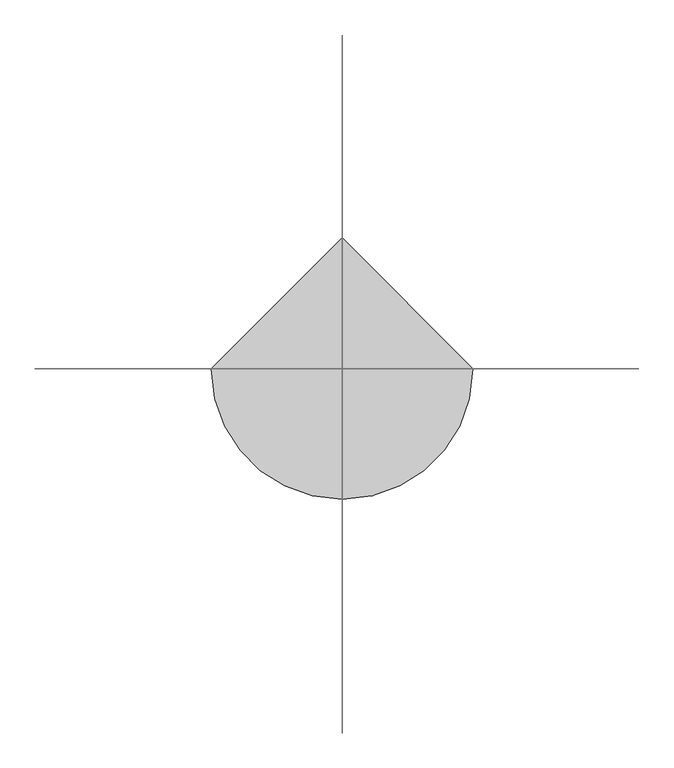
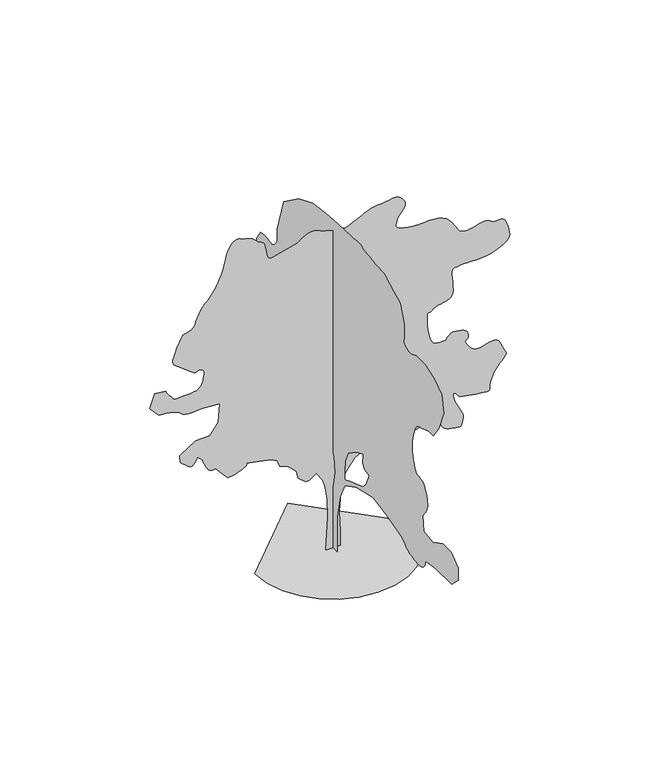
"""IFC4 building model written with IfcOpenShell, lengths in millimetres: geographic element geometry, RPC 木 - 落葉樹 : サンザシ - 7.4 メートル."""

from ifc_helpers import new_model, si_unit, origin, place, context, project, spatial, triangles, source, transform, mapped, element, save


def geographic_element_c28d403f(model_context):
    return source(origin(), model_context, "Body", "Tessellation", [
        triangles([(154.5387321, 0.0003833, 0.0187505), (-149.642156, 0.0003833, 0.0187505), (-106.1871776, 0.0003405, 717.0148825), (-117.051113, 0.0003185, 1086.3780928), (-160.5051012, 0.0003017, 1368.8308376), (-203.9600796, 0.0002913, 1542.6492977), (-345.1849986, 0.0002797, 1738.1941933), (-486.4138418, 0.0002855, 1640.4205101), (-562.4586551, 0.0002862, 1629.557365), (-714.5482452, 0.0002784, 1759.9204834), (-758.0034416, 0.000268, 1933.7389435), (-910.0929955, 0.000259, 2085.8284973), (-1094.7746733, 0.0002544, 2161.8732742), (-1149.0930147, 0.0002467, 2292.2365379), (-1268.5930607, 0.0002428, 2357.4181698), (-1518.4538269, 0.0002395, 2411.7365112), (-1768.3170639, 0.0002369, 2455.1893822), (-1766.353521, 0.0002375, 2445.7838516), (-1766.5756004, 0.0002381, 2435.806263), (-1771.1684887, 0.0002388, 2424.6889183), (-1782.3178082, 0.0002395, 2411.8623756), (-1802.2065651, 0.0002404, 2396.7539955), (-1833.0250328, 0.0002415, 2378.7966614), (-1876.9538921, 0.0002428, 2357.4181698), (-1925.9491573, 0.000244, 2336.6735058), (-1970.9560032, 0.000245, 2320.4872845), (-2012.6351452, 0.0002457, 2308.1046101), (-2051.6577633, 0.0002463, 2298.760849), (-2088.6823929, 0.0002467, 2291.6987801), (-2124.375127, 0.000247, 2286.1562405), (-2159.4067097, 0.0002473, 2281.3732475), (-2278.906683, 0.0002395, 2411.7365112), (-2409.2698013, 0.0002305, 2563.8260651), (-2434.8615532, 0.0002307, 2559.4600525), (-2460.3567993, 0.0002309, 2556.7959709), (-2485.6575806, 0.0002308, 2557.5607498), (-2510.6941338, 0.0002305, 2563.4560295), (-2535.3362343, 0.0002297, 2576.1840317), (-2559.4847603, 0.0002285, 2597.4713951), (-2583.0908775, 0.0002266, 2628.995343), (-2604.4767815, 0.0002244, 2664.9841347), (-2622.4341156, 0.0002224, 2698.6785896), (-2637.5299965, 0.0002205, 2730.4740326), (-2650.3565392, 0.0002187, 2760.7646255), (-2661.4814415, 0.000217, 2789.8959869), (-2671.4465309, 0.0002153, 2818.2872772), (-2680.8692116, 0.0002136, 2846.2838242), (-2778.6231285, 0.0002078, 2944.0624489), (-2843.8171143, 0.0002136, 2846.2838242), (-2855.5832565, 0.0002147, 2827.9317467), (-2868.2371353, 0.0002157, 2811.3065987), (-2882.568528, 0.0002165, 2798.1097298), (-2899.4898788, 0.000217, 2790.0192352), (-2919.8150917, 0.0002171, 2788.7858803), (-2944.4324844, 0.0002166, 2796.1118866), (-2974.180378, 0.0002156, 2813.6991852), (-3007.1350525, 0.0002141, 2838.6124901), (-3039.7443993, 0.0002125, 2865.4498055), (-3070.2323639, 0.0002109, 2892.0897491), (-3096.9461403, 0.0002094, 2916.4356468), (-3118.1349632, 0.0002083, 2936.4158226), (-3132.0963203, 0.0002074, 2949.9330208), (-3137.1282806, 0.0002072, 2954.9158562), (-3147.9813972, 0.0001981, 3107.0103516), (-2822.0858826, 0.0001858, 3313.4207176), (-2528.7747162, 0.0001851, 3324.2741249), (-2354.9514599, 0.0001715, 3552.4157227), (-2322.3594086, 0.0001482, 3943.5055138), (-2680.8692116, 0.0001463, 3976.0901527), (-2757.4098885, 0.0001468, 3967.0866325), (-2832.3471748, 0.0001472, 3960.0074135), (-2904.0529724, 0.0001474, 3956.702092), (-2970.924472, 0.0001473, 3959.1193863), (-3031.3082863, 0.0001467, 3969.1338913), (-3083.6263138, 0.0001455, 3988.6452003), (-3126.2748734, 0.0001437, 4019.5526161), (-3169.2196358, 0.0001417, 4052.6799545), (-3222.4253998, 0.0001402, 4078.3824554), (-3284.1908157, 0.000139, 4097.9431801), (-3352.7886635, 0.0001382, 4112.5457771), (-3426.5173027, 0.0001375, 4123.4238922), (-3503.6745117, 0.000137, 4131.8600052), (-3582.5336517, 0.0001366, 4139.0377647), (-3767.2127861, 0.0001243, 4345.4484215), (-3658.5810448, 0.0001074, 4627.9061806), (-3441.3172714, 0.0001087, 4606.1746582), (-3427.2817909, 0.0001103, 4580.6201134), (-3412.8765656, 0.0001118, 4555.3367729), (-3397.7065613, 0.0001132, 4530.6455475), (-3381.3773254, 0.0001147, 4506.7929337), (-3363.5432396, 0.000116, 4484.0748436), (-3343.8098511, 0.0001173, 4462.812188), (-3321.807415, 0.0001184, 4443.2267555), (-3305.3052246, 0.0001195, 4424.7517204), (-3297.5600578, 0.0001206, 4407.2382545), (-3291.3194504, 0.0001215, 4391.624382), (-3279.3806442, 0.0001223, 4378.8716721), (-3254.5167549, 0.0001228, 4369.9175674), (-3209.5000259, 0.0001231, 4365.699511), (-3137.1282806, 0.000123, 4367.1796532), (-3056.9122467, 0.0001227, 4371.8415779), (-2991.4964722, 0.0001224, 4376.5035027), (-2938.4383736, 0.0001221, 4381.1410103), (-2895.2718224, 0.0001219, 4385.802935), (-2859.529818, 0.0001216, 4390.4648598), (-2828.6965256, 0.0001213, 4395.1270752), (-2800.3546509, 0.000121, 4399.7642921), (-2772.6046005, 0.0001198, 4420.8295761), (-2746.0137817, 0.0001185, 4442.5608078), (-2721.6925919, 0.0001171, 4465.6242256), (-2700.775264, 0.0001156, 4490.6607788), (-2684.4460281, 0.000114, 4518.3861214), (-2673.7899925, 0.0001121, 4549.4167854), (-2669.9913872, 0.00011, 4584.4434265), (-2666.1433662, 0.0001077, 4623.3427963), (-2657.7072533, 0.0001053, 4664.1414688), (-2649.4688026, 0.0001029, 4704.7427696), (-2646.1878983, 0.0001006, 4743.0747322), (-2652.5767525, 9.85e-05, 4777.0159744), (-2673.419957, 9.69e-05, 4804.5192375), (-2713.4538506, 9.58e-05, 4823.4631393), (-2753.6112831, 9.55e-05, 4827.7059036), (-2778.0065964, 9.61e-05, 4818.8259224), (-2796.1118866, 9.68e-05, 4806.3444168), (-2817.4730827, 9.72e-05, 4799.7584816), (-2851.5378639, 9.67e-05, 4808.5646301), (-2907.8518684, 9.47e-05, 4842.2590851), (-2995.9116096, 9.06e-05, 4910.363649), (-3093.616111, 8.61e-05, 4986.2136703), (-3172.3275856, 8.27e-05, 5042.3055954), (-3231.6507088, 8.01e-05, 5086.8040421), (-3271.1913185, 7.76e-05, 5127.8986267), (-3290.6040871, 7.49e-05, 5173.7045517), (-3289.4939804, 7.14e-05, 5232.460849), (-3267.4915443, 6.66e-05, 5312.3065567), (-3236.1646774, 6.15e-05, 5397.8257553), (-3207.1321472, 5.73e-05, 5469.6550919), (-3179.9742119, 5.37e-05, 5530.0886124), (-3154.3702515, 5.06e-05, 5581.3953644), (-3129.876107, 4.8e-05, 5625.8688126), (-3106.1470322, 4.56e-05, 5665.7797485), (-3082.8121193, 4.33e-05, 5703.3960571), (-3038.7575409, 4.28e-05, 5712.9669846), (-2995.7389458, 4.21e-05, 5724.0424713), (-2954.817025, 4.13e-05, 5738.1764923), (-2917.0277618, 4.01e-05, 5756.8736069), (-2883.4318474, 3.87e-05, 5781.6389557), (-2855.0652649, 3.67e-05, 5814.0015152), (-2832.9392899, 3.43e-05, 5855.4908432), (-2817.1771706, 3.18e-05, 5897.3749146), (-2805.2139473, 2.97e-05, 5932.401265), (-2794.1878761, 2.78e-05, 5964.3940796), (-2781.2625023, 2.58e-05, 5997.126384), (-2763.5766632, 2.36e-05, 6034.4473618), (-2738.3180305, 2.09e-05, 6080.10504), (-2702.5760262, 1.74e-05, 6137.9486023), (-2665.3294624, 1.43e-05, 6190.7349152), (-2634.7426666, 1.22e-05, 6225.120607), (-2606.8199524, 1.07e-05, 6250.5516129), (-2577.5406349, 9.2e-06, 6276.5506073), (-2542.9581528, 7e-06, 6312.612941), (-2499.0515305, 3.7e-06, 6368.2607071), (-2441.8593819, -1.3e-06, 6452.9910004), (-2383.0122471, -7.2e-06, 6551.6820694), (-2335.5683407, -1.27e-05, 6643.9107422), (-2297.6237091, -1.79e-05, 6731.2059952), (-2267.2812298, -2.29e-05, 6815.0723877), (-2242.6392746, -2.78e-05, 6897.0400589), (-2221.8008663, -3.27e-05, 6978.6368225), (-2202.8594353, -3.76e-05, 7061.3439835), (-2179.771455, -4.26e-05, 7144.3970535), (-2148.5114445, -4.72e-05, 7222.8858673), (-2110.218869, -5.14e-05, 7292.248494), (-2066.0359554, -5.47e-05, 7347.9212585), (-2017.1023144, -5.69e-05, 7385.3654846), (-1964.559882, -5.78e-05, 7399.9924988), (-1909.5434727, -5.7e-05, 7387.2647873), (-1854.9734024, -5.56e-05, 7363.9795807), (-1802.870042, -5.47e-05, 7347.3538513), (-1753.0508446, -5.38e-05, 7333.3924942), (-1705.3209091, -5.29e-05, 7318.0992416), (-1659.4902763, -5.17e-05, 7297.4778259), (-1615.3714577, -4.99e-05, 7267.5325607), (-1572.7721684, -4.73e-05, 7224.3165939), (-1533.465992, -4.5e-05, 7185.4666397), (-1499.1028278, -4.38e-05, 7165.0673035), (-1469.2981064, -4.31e-05, 7153.6220718), (-1443.6768505, -4.24e-05, 7141.5850159), (-1421.8543453, -4.11e-05, 7119.4834579), (-1403.4529976, -3.86e-05, 7077.797049), (-1388.0905632, -3.44e-05, 7007.0281128), (-1375.106036, -2.96e-05, 6926.4673325), (-1362.6913868, -2.57e-05, 6861.273056), (-1348.7547375, -2.27e-05, 6810.9284546), (-1331.2092968, -2.05e-05, 6774.8167053), (-1307.9610065, -1.92e-05, 6752.3948181), (-1276.9229301, -1.86e-05, 6743.0703873), (-1236.0010094, -1.88e-05, 6746.3021667), (-736.2770788, -2.66e-05, 6876.6651398), (-678.0613008, -2.91e-05, 6918.1050522), (-619.7543221, -3.14e-05, 6956.6835114), (-561.2549131, -3.33e-05, 6989.5396454), (-502.4718369, -3.48e-05, 7013.8858337), (-443.3064076, -3.55e-05, 7026.7862091), (-383.6674244, -3.55e-05, 7025.4787308), (-323.4585995, -3.44e-05, 7007.0281128), (-263.8837293, -3.28e-05, 6981.3256119), (-206.018257, -3.15e-05, 6959.5943802), (-149.57827, -3.04e-05, 6941.1931778), (-94.2786203, -2.95e-05, 6925.4557663), (-39.8339149, -2.87e-05, 6911.6914902), (14.0404504, -2.79e-05, 6899.2846893), (67.6297655, -2.72e-05, 6887.5429642), (263.1757965, -2.6e-05, 6865.8117325), (567.3549768, -3.37e-05, 6996.1752869), (611.7598246, -3.54e-05, 7023.9247559), (657.2106113, -3.7e-05, 7050.5155746), (704.7506601, -3.84e-05, 7074.8367645), (755.4257647, -3.97e-05, 7095.7540924), (810.2819366, -4.06e-05, 7112.0833282), (870.3648972, -4.13e-05, 7122.7396545), (936.7181871, -4.15e-05, 7126.5382599), (1008.7398811, -4.18e-05, 7131.6687607), (1083.2330812, -4.25e-05, 7143.6319839), (1157.346508, -4.33e-05, 7157.3224274), (1228.2285187, -4.39e-05, 7167.583429), (1293.0303772, -4.4e-05, 7169.2856506), (1348.9002228, -4.33e-05, 7157.3224274), (1392.9893921, -4.15e-05, 7126.5382599), (1427.384531, -3.91e-05, 7086.4302429), (1455.3195992, -3.69e-05, 7049.1836792), (1475.6522243, -3.48e-05, 7013.6637543), (1487.2455574, -3.27e-05, 6978.6862381), (1488.9550461, -3.06e-05, 6943.1418961), (1479.6432598, -2.83e-05, 6905.8953323), (1458.1685532, -2.6e-05, 6865.8117325), (1431.5655258, -2.38e-05, 6829.329657), (1407.6216385, -2.21e-05, 6801.3825256), (1386.3367458, -2.08e-05, 6778.5903122), (1367.713464, -1.95e-05, 6757.5003204), (1351.7516476, -1.81e-05, 6734.6836899), (1338.4489712, -1.65e-05, 6706.761557), (1327.8052895, -1.43e-05, 6670.254483), (1316.5943459, -1.2e-05, 6630.8865372), (1304.6235649, -9.9e-06, 6596.0822662), (1296.4515347, -8e-06, 6565.0760193), (1296.641494, -6.4e-06, 6537.1038895), (1309.7543564, -4.8e-06, 6511.426387), (1340.3482738, -3.4e-06, 6487.2528625), (1392.9893921, -2e-06, 6463.8444077), (1459.1822994, -8e-07, 6443.7409836), (1526.1375149, 1e-07, 6429.3354675), (1591.9529743, 6e-07, 6419.6662903), (1654.727195, 1e-06, 6413.8201355), (1712.5605835, 1.2e-06, 6410.8110168), (1763.5538372, 1.2e-06, 6409.7012009), (1805.805328, 1.2e-06, 6409.528537), (1853.5354088, 1.1e-06, 6412.1673294), (1918.9389748, 8e-07, 6417.2734131), (1997.0730137, 6e-07, 6420.652858), (2082.9993095, 7e-07, 6418.161731), (2171.7770302, 1.5e-06, 6405.5816849), (2258.4628727, 3.1e-06, 6378.7443695), (2338.1213825, 5.8e-06, 6333.4808533), (2404.5683441, 9.3e-06, 6273.6641556), (2457.3351814, 1.32e-05, 6208.69254), (2500.0380981, 1.71e-05, 6142.7831909), (2536.2733864, 2.09e-05, 6080.10504), (2569.6475121, 2.42e-05, 6024.8520172), (2603.7861259, 2.68e-05, 5981.1674744), (2642.2907524, 2.84e-05, 5953.2691772), (2685.4820114, 2.93e-05, 5939.3822342), (2730.9179008, 2.96e-05, 5934.0784882), (2778.2778008, 2.95e-05, 5935.879541), (2827.1425507, 2.9e-05, 5943.3779205), (2877.1418243, 2.83e-05, 5955.1684799), (2927.930294, 2.75e-05, 5969.7960754), (2979.0643822, 2.65e-05, 5985.8538162), (3025.5115471, 2.6e-05, 5994.8817535), (3071.169516, 2.55e-05, 6002.2080505), (3115.3229256, 2.53e-05, 6006.1054871), (3157.2067062, 2.54e-05, 6004.8718414), (3196.0322433, 2.58e-05, 5996.7810562), (3231.0588844, 2.68e-05, 5980.1559082), (3261.5221413, 2.84e-05, 5953.2691772), (3295.4880913, 2.96e-05, 5933.5360794), (3338.9261375, 2.97e-05, 5932.4262634), (3388.0865089, 2.93e-05, 5939.3078201), (3439.1464737, 2.9e-05, 5943.5011688), (3488.3071358, 2.96e-05, 5934.4238159), (3531.745182, 3.15e-05, 5901.3955994), (3565.711132, 3.56e-05, 5833.7596115), (3592.474324, 4.06e-05, 5749.3008133), (3614.8717941, 4.52e-05, 5672.809552), (3629.8444267, 4.92e-05, 5604.3102448), (3634.3831032, 5.28e-05, 5543.7784744), (3625.4042908, 5.6e-05, 5491.2386581), (3599.9238693, 5.86e-05, 5446.6657974), (3554.833017, 6.08e-05, 5410.0854721), (3500.9613052, 6.27e-05, 5377.6484985), (3448.4211983, 6.46e-05, 5346.1742569), (3393.2173004, 6.64e-05, 5316.5987366), (3331.353344, 6.8e-05, 5289.8602524), (3258.8580597, 6.93e-05, 5266.9197922), (3171.7354706, 7.04e-05, 5248.7406693), (3065.9895996, 7.12e-05, 5236.2594543), (2962.6116074, 7.15e-05, 5229.969722), (2881.4584213, 7.16e-05, 5228.4151657), (2816.8565506, 7.16e-05, 5229.722644), (2763.0586716, 7.14e-05, 5231.9672745), (2714.4160011, 7.14e-05, 5233.2503357), (2665.2059235, 7.14e-05, 5231.6963608), (2609.7061134, 7.18e-05, 5225.4060471), (2556.2041466, 7.22e-05, 5218.7215714), (2515.6522614, 7.25e-05, 5214.5032242), (2486.2741127, 7.28e-05, 5208.5832367), (2466.4250336, 7.35e-05, 5196.7682602), (2454.3580376, 7.48e-05, 5174.8887817), (2448.3714844, 7.7e-05, 5138.752034), (2446.7558853, 8.02e-05, 5084.1896667), (2451.1265488, 8.46e-05, 5010.8557709), (2460.4384804, 8.97e-05, 4925.9528137), (2468.9827263, 9.5e-05, 4836.4626366), (2471.0794006, 0.0001002, 4749.4632957), (2461.008213, 0.0001048, 4671.960759), (2433.0731449, 0.0001084, 4610.9848297), (2381.5741081, 0.0001107, 4573.5900192), (2319.0219669, 0.0001118, 4553.8569214), (2261.6004719, 0.0001127, 4539.4514053), (2209.119809, 0.0001134, 4527.6855537), (2161.3898735, 0.0001141, 4515.9441193), (2118.2207062, 0.000115, 4501.5388939), (2079.4201675, 0.0001161, 4481.8055054), (2044.8029491, 0.0001178, 4454.0801628), (2014.8403885, 0.0001191, 4432.4474716), (1990.0109447, 0.0001195, 4426.0342003), (1970.119717, 0.0001195, 4424.7270126), (1954.9818329, 0.0001199, 4418.4861145), (1944.4023914, 0.0001212, 4397.2481667), (1938.1937588, 0.0001239, 4350.8995422), (1936.1661209, 0.0001288, 4269.4010284), (1940.60117, 0.000135, 4165.1844246), (1953.0184353, 0.0001412, 4060.746032), (1972.08326, 0.0001472, 3961.2654762), (1996.4711609, 0.0001525, 3871.8488411), (2024.8500973, 0.0001569, 3797.6516258), (2055.8881737, 0.0001601, 3743.7796234), (2088.2581455, 0.0001618, 3715.3636253), (2125.4406143, 0.0001625, 3704.510218), (2168.895956, 0.0001628, 3698.9602661), (2214.2504551, 0.0001629, 3697.4062912), (2257.1359188, 0.0001628, 3698.5163979), (2293.1763062, 0.0001627, 3700.9584), (2318.0082207, 0.0001625, 3703.4004021), (2327.2582375, 0.0001625, 3704.510218), (2330.7090443, 0.000162, 3712.8230827), (2341.5721893, 0.0001607, 3733.8883667), (2360.60751, 0.0001591, 3761.7863731), (2388.5745529, 0.0001573, 3790.6462395), (2426.2331554, 0.0001559, 3814.5729767), (2474.3355972, 0.0001551, 3827.6463066), (2533.6587204, 0.0001554, 3823.9953667), (2594.8320213, 0.0001561, 3811.5141518), (2647.8159966, 0.0001568, 3799.9947968), (2692.4379822, 0.0001576, 3786.3787674), (2728.5006065, 0.0001587, 3767.6322372), (2755.8559135, 0.0001603, 3740.6963814), (2774.2571159, 0.0001626, 3702.5614998), (2783.5318405, 0.0001657, 3650.1943474), (2780.0538551, 0.0001685, 3602.8344475), (2764.9579742, 0.0001701, 3575.9971321), (2745.3231262, 0.000171, 3560.9750839), (2728.1552788, 0.0001717, 3548.9624451), (2720.5086525, 0.0001728, 3531.2518982), (2729.3639259, 0.0001747, 3499.1111275), (2761.8006088, 0.000178, 3443.7839813), (2805.9293106, 0.0001816, 3384.041407), (2846.0370369, 0.0001841, 3342.3547073), (2883.5056801, 0.0001857, 3315.4926842), (2919.6671356, 0.0001866, 3300.2485565), (2955.8035927, 0.000187, 3293.3420013), (2993.2722359, 0.0001871, 3291.565947), (3033.3802528, 0.0001871, 3291.6894859), (3083.0836143, 0.0001865, 3301.1859993), (3144.9475708, 0.0001852, 3322.4733627), (3213.8169136, 0.0001839, 3344.6978783), (3284.6099762, 0.0001832, 3357.0558449), (3352.1718407, 0.0001837, 3348.6938553), (3411.3720062, 0.0001861, 3308.7835007), (3457.0791, 0.000191, 3226.4955002), (3493.1417244, 0.0001964, 3135.4754745), (3524.8383362, 0.0002002, 3071.6383827), (3549.1351089, 0.0002028, 3027.5343887), (3562.9732178, 0.0002047, 2995.8130692), (3563.3429626, 0.0002063, 2969.0004616), (3547.1369751, 0.0002081, 2939.7458519), (3511.3952614, 0.0002104, 2900.5996948), (3469.3632339, 0.000213, 2857.4331436), (3435.54524, 0.0002153, 2820.3839516), (3408.510553, 0.0002173, 2788.4158447), (3386.9272774, 0.0002191, 2760.5178383), (3369.4385193, 0.0002207, 2735.6786568), (3354.6879662, 0.0002222, 2712.886734), (3341.2940163, 0.0002237, 2691.0813789), (3337.963987, 0.0002234, 2693.4739655), (3333.4253105, 0.0002233, 2692.0926544), (3326.4940475, 0.0002237, 2683.2620888), (3315.9612602, 0.0002247, 2663.2327881), (3300.6185921, 0.0002267, 2628.2799797), (3279.2326881, 0.0002298, 2574.6547646), (3250.668734, 0.0002343, 2498.6567871), (3229.134874, 0.000239, 2421.0802723), (3223.3628426, 0.0002424, 2363.6563065), (3223.8561264, 0.0002448, 2323.9084419), (3221.1429199, 0.0002462, 2299.3627018), (3205.6767128, 0.0002469, 2287.5499054), (3167.9862808, 0.000247, 2285.9957851), (3098.5742386, 0.0002467, 2292.2365379), (3013.9183594, 0.0002461, 2301.8638573), (2936.0952026, 0.0002455, 2312.0635254), (2863.9696632, 0.0002448, 2322.7368565), (2796.4077988, 0.0002442, 2333.7899609), (2732.2745041, 0.0002435, 2345.1292397), (2670.4352554, 0.0002428, 2356.6583324), (2609.7061134, 0.0002421, 2368.2813148), (2570.6340797, 0.0002393, 2416.1074654), (2534.497332, 0.0002368, 2457.5648186), (2504.2314468, 0.0002351, 2486.2988205), (2482.8208351, 0.0002345, 2495.9188728), (2473.2007828, 0.0002355, 2480.0829208), (2478.3068665, 0.0002383, 2432.4170803), (2501.0740814, 0.0002434, 2346.5548794), (2537.5067413, 0.0002493, 2247.0398781), (2578.280706, 0.0002545, 2161.0173672), (2618.5119713, 0.0002589, 2086.0184566), (2653.2179924, 0.0002629, 2019.5690243), (2677.4900574, 0.0002665, 1959.2023602), (2686.3453308, 0.0002699, 1902.4468128), (2674.9000992, 0.0002732, 1846.8285507), (2657.8799171, 0.0002761, 1797.4532215), (2649.2467232, 0.0002784, 1760.4261211), (2642.6854958, 0.0002799, 1734.8048653), (2631.9553368, 0.0002808, 1719.6325356), (2610.7668045, 0.0002811, 1713.9641315), (2572.8540024, 0.0002809, 1716.8452057), (2511.9274887, 0.0002803, 1727.3284321), (2443.842691, 0.0002795, 1740.8853081), (2387.5286865, 0.0002787, 1754.6319981), (2341.4761196, 0.0002778, 1770.0880314), (2304.1677864, 0.0002767, 1788.7730827), (2274.0793613, 0.0002753, 1812.2113323), (2249.6914604, 0.0002735, 1841.9198387), (2229.4845543, 0.0002713, 1879.4204567), (2216.7196358, 0.0002688, 1919.8663891), (2212.5089916, 0.0002666, 1956.8910187), (2212.0970982, 0.0002647, 1989.7346535), (2210.735408, 0.000263, 2017.6376015), (2203.6708683, 0.0002617, 2039.8400253), (2186.1575478, 0.0002608, 2055.5797623), (2153.4397774, 0.0002603, 2064.1022072), (2114.7033337, 0.00026, 2067.8070683), (2081.6697395, 0.0002599, 2069.802586), (2053.3870182, 0.0002599, 2070.372464), (2028.9029022, 0.0002599, 2069.802586), (2007.2726818, 0.00026, 2068.3768009), (1987.5392933, 0.0002601, 2066.3812832), (1968.7581722, 0.0002603, 2064.1022072), (1708.0317902, 0.0002661, 1966.328524), (1534.2133301, 0.000259, 2085.8284973), (1341.0438709, 0.0002626, 2015.5359856), (1370.1210205, 0.0002638, 1997.904213), (1395.1328659, 0.000265, 1979.658379), (1412.0148296, 0.0002662, 1960.1839863), (1416.7014622, 0.0002676, 1938.8646481), (1405.1278954, 0.0002691, 1915.0860123), (1373.2314411, 0.0002707, 1888.2338722), (1316.9446152, 0.0002726, 1857.6916958), (1256.1339375, 0.0002741, 1830.8987091), (1209.5731894, 0.0002751, 1814.9345673), (1171.566861, 0.0002755, 1808.6643105), (1136.4119574, 0.0002753, 1810.9433865), (1098.4055563, 0.0002748, 1820.6374168), (1051.847279, 0.0002738, 1836.5992332), (991.0366013, 0.0002726, 1857.6916958), (708.5813856, 0.0002674, 1944.6020885), (447.8549672, 0.0002758, 1803.3756798), (252.3101443, 0.0002913, 1542.6492977), (187.1297842, 0.0003023, 1357.9676926), (165.4019135, 0.0003159, 1129.8333618), (132.8118606, 0.0003386, 749.6069338), (154.5387321, 0.0003658, 293.3357107), (-0.0001194, -152.9413187, 0.0155948), (-0.0001194, 162.1054759, 0.0156136), (-9.83e-05, 172.6070515, 682.6172728), (-8.43e-05, 225.1146749, 1029.1687941), (-7.02e-05, 393.1394116, 1375.7202427), (-6.32e-05, 550.6630451, 1606.752943), (-5.62e-05, 823.7030651, 1795.7809399), (-4.21e-05, 1296.2739292, 2005.8124512), (-2.81e-05, 1852.8569618, 2068.8208145), (-2.81e-05, 2178.4048233, 1869.2924412), (-2.81e-05, 2419.9406616, 1837.7881142), (-2.11e-05, 2556.4506432, 2100.3276123), (-1.4e-05, 2776.9953209, 2131.831794), (-7e-06, 3239.0508385, 2163.3359756), (0.0, 3512.1106247, 2184.3396355), (7e-06, 3648.6156647, 2289.3554638), (7e-06, 3638.1322929, 2457.3796555), (1.4e-05, 3806.1368637, 2562.3953384), (1.4e-05, 3853.1514359, 2571.5221069), (1.4e-05, 3898.5873253, 2581.3886559), (1.4e-05, 3940.8908478, 2592.7106392), (2.11e-05, 3978.5074471, 2606.2281281), (2.11e-05, 4009.907856, 2622.70532), (2.11e-05, 4033.4645576, 2642.8581596), (2.11e-05, 4047.672702, 2667.401429), (2.11e-05, 4056.0593994, 2696.8534103), (2.11e-05, 4063.3606979, 2730.7205292), (2.11e-05, 4069.7245537, 2768.2632957), (2.81e-05, 4075.348629, 2808.7410576), (2.81e-05, 4080.4300049, 2851.4146156), (2.81e-05, 4085.166053, 2895.5677345), (2.81e-05, 4089.6800217, 2940.4609245), (3.51e-05, 3911.1673714, 3160.9808945), (2.81e-05, 3522.5937057, 3181.9967628), (2.11e-05, 3291.565947, 3013.967775), (2.11e-05, 3277.4566338, 3011.1804451), (2.11e-05, 3240.3827339, 3004.5203865), (2.11e-05, 3188.2373703, 2996.6022652), (1.4e-05, 3128.9389549, 2989.9669144), (1.4e-05, 3070.3556122, 2987.1795845), (1.4e-05, 3020.4301712, 2990.8058167), (1.4e-05, 2987.0316284, 3003.4596954), (1.4e-05, 2964.2149979, 3024.8208916), (1.4e-05, 2940.8556679, 3052.2750298), (1.4e-05, 2917.0277618, 3084.7361298), (1.4e-05, 2892.854528, 3121.2676208), (2.11e-05, 2868.3850914, 3160.8329384), (2.11e-05, 2843.7432816, 3202.4208069), (2.11e-05, 2819.0026405, 3244.9955338), (2.81e-05, 2766.4872414, 3507.5472404), (3.51e-05, 2987.0316284, 3675.5515205), (4.92e-05, 3155.060907, 3959.0946785), (4.92e-05, 2882.0011208, 4211.1385963), (4.21e-05, 2598.4579628, 4116.6158775), (3.51e-05, 2419.9406616, 3969.602758), (3.51e-05, 2220.4096722, 4106.1325058), (4.21e-05, 2220.4096722, 4337.1602646), (5.62e-05, 2409.4375237, 4547.1968628), (5.62e-05, 2449.8216866, 4569.6681656), (5.62e-05, 2489.4808937, 4591.9420967), (5.62e-05, 2527.6401924, 4613.8707001), (5.62e-05, 2563.6286934, 4635.2318962), (5.62e-05, 2596.6574913, 4655.8780197), (6.32e-05, 2626.0106415, 4675.5867004), (6.32e-05, 2650.973362, 4694.2099823), (6.32e-05, 2670.4105476, 4720.1839783), (6.32e-05, 2684.347197, 4760.4646591), (6.32e-05, 2693.6960449, 4812.7085632), (7.02e-05, 2699.3445374, 4874.4736885), (7.02e-05, 2702.2554062, 4943.4418625), (7.02e-05, 2703.3405144, 5017.1455032), (7.02e-05, 2703.4887611, 5093.2670197), (7.73e-05, 2566.9587227, 5303.3036179), (7.73e-05, 2562.0253029, 5304.437851), (7.73e-05, 2548.1133614, 5307.2254715), (7.73e-05, 2526.4562531, 5310.7525818), (7.73e-05, 2498.3855827, 5314.0826111), (7.73e-05, 2465.1620293, 5316.3028244), (7.73e-05, 2428.0830425, 5316.5249039), (7.73e-05, 2388.4364799, 5313.811116), (7.73e-05, 2346.3082375, 5307.7184647), (7.02e-05, 2302.157444, 5299.7759262), (7.02e-05, 2257.8241035, 5292.0304688), (7.02e-05, 2215.1458946, 5286.4808075), (7.02e-05, 2175.9555542, 5285.1733292), (7.02e-05, 2142.0930862, 5290.106749), (7.02e-05, 2115.39646, 5303.3036179), (7.02e-05, 2093.8105682, 5322.2228119), (7.02e-05, 2073.8799534, 5342.794812), (7.02e-05, 2055.325708, 5364.7481232), (7.02e-05, 2037.874157, 5387.8112503), (7.02e-05, 2021.2487183, 5411.6888626), (7.02e-05, 2005.1735367, 5436.1083023), (7.02e-05, 1989.3769718, 5460.8248169), (8.43e-05, 1978.8739792, 5723.3518158), (9.83e-05, 1758.3418007, 6458.4668289), (0.0001054, 1222.7624279, 6847.0402039), (0.0001054, 718.6873095, 7057.0523849), (9.83e-05, 256.6194016, 7120.0752823), (9.13e-05, -194.9473848, 7151.5751038), (8.43e-05, -636.0121233, 7172.5906815), (8.43e-05, -674.6820013, 7174.7858963), (8.43e-05, -731.9036539, 7179.9169785), (8.43e-05, -800.516399, 7185.8119675), (8.43e-05, -873.3545403, 7190.2029785), (8.43e-05, -943.2523813, 7190.9430496), (7.73e-05, -1003.0467693, 7185.8119675), (7.73e-05, -1045.5745514, 7172.5906815), (7.73e-05, -1089.3258053, 7155.7928696), (7.73e-05, -1152.5488358, 7141.2396881), (7.73e-05, -1227.7129978, 7128.4869781), (7.73e-05, -1307.2851757, 7117.2144104), (7.02e-05, -1383.7344337, 7107.0516586), (7.02e-05, -1449.5302723, 7097.628978), (7.02e-05, -1497.1394302, 7088.5760422), (7.02e-05, -1540.7992653, 7082.3107269), (7.02e-05, -1596.950489, 7079.7457672), (7.02e-05, -1661.367342, 7078.0929611), (6.32e-05, -1729.8272621, 7074.6146851), (6.32e-05, -1798.1020191, 7066.5244812), (6.32e-05, -1861.9689056, 7051.0829819), (6.32e-05, -1917.2024529, 7025.5531448), (6.32e-05, -1970.689595, 6993.1411697), (5.62e-05, -2031.3424335, 6959.0519714), (5.62e-05, -2097.9645298, 6923.6058792), (5.62e-05, -2169.3620613, 6887.049971), (4.92e-05, -2244.3438217, 6849.6551605), (4.92e-05, -2321.710611, 6811.7179413), (4.92e-05, -2400.2739841, 6773.509227), (3.51e-05, -2547.2994576, 6405.9764282), (2.11e-05, -2536.791378, 6069.9178711), (2.11e-05, -2528.1828918, 6054.0822098), (2.11e-05, -2521.9667015, 6037.8018082), (2.11e-05, -2520.5362656, 6020.5848358), (2.11e-05, -2526.2588814, 6002.0103882), (2.11e-05, -2541.5521339, 5981.5866348), (2.11e-05, -2568.7594849, 5958.8688354), (2.11e-05, -2610.2979378, 5933.3878326), (2.11e-05, -2660.1245476, 5913.1367432), (1.4e-05, -2710.4938568, 5904.9721252), (1.4e-05, -2761.307325, 5906.9452606), (1.4e-05, -2812.490538, 5916.9847641), (1.4e-05, -2863.9696632, 5933.0919205), (1.4e-05, -2915.621743, 5953.2447601), (1.4e-05, -2967.3476555, 5975.3951523), (7e-06, -3292.8981331, 5975.3951523), (0.0, -3618.44832, 5870.3893524), (-7e-06, -3881.0000267, 5681.3689133), (-2.11e-05, -3943.9987976, 5313.811116), (-2.81e-05, -3765.4861473, 4872.7470497), (-3.51e-05, -3576.4410004, 4610.195343), (-3.51e-05, -3542.4259254, 4610.0226791), (-3.51e-05, -3506.8565849, 4608.7401993), (-3.51e-05, -3468.1545868, 4605.2375061), (-3.51e-05, -3424.7659561, 4598.4541992), (-3.51e-05, -3375.136718, 4587.2307564), (-3.51e-05, -3317.7126068, 4570.531485), (-2.81e-05, -3250.8908134, 4547.1968628), (-2.81e-05, -3183.8713577, 4524.72556), (-2.81e-05, -3126.2254578, 4508.8649002), (-2.81e-05, -3077.0156708, 4495.9395264), (-2.81e-05, -3035.3536789, 4482.2740814), (-2.81e-05, -3000.30233, 4464.2182068), (-2.81e-05, -2970.9488892, 4438.0715469), (-2.81e-05, -2946.3564949, 4400.1590355), (-3.51e-05, -2922.2818016, 4345.7690414), (-3.51e-05, -2896.57901, 4276.1105026), (-3.51e-05, -2871.3945007, 4196.5357086), (-3.51e-05, -2848.9970306, 4112.3731133), (-4.21e-05, -2831.533271, 4028.950589), (-4.21e-05, -2821.247271, 3951.5713005), (-4.21e-05, -2820.334536, 3885.5881187), (-4.92e-05, -2829.0665611, 3818.100087), (-4.92e-05, -2845.1245926, 3737.9581764), (-4.92e-05, -2866.9052399, 3653.0310928), (-5.62e-05, -2892.706572, 3571.2116684), (-5.62e-05, -2920.9004906, 3500.4430229), (-6.32e-05, -2949.8344803, 3448.5691544), (-6.32e-05, -2977.855735, 3423.5326012), (-6.32e-05, -3011.22957, 3416.5519226), (-6.32e-05, -3054.5196602, 3411.396714), (-6.32e-05, -3103.5076584, 3404.786071), (-6.32e-05, -3153.9755081, 3393.3899643), (-6.32e-05, -3201.656028, 3373.9280708), (-7.02e-05, -3242.3808678, 3343.0700706), (-7.02e-05, -3271.9066818, 3297.5106422), (-7.02e-05, -3294.7974358, 3244.6993309), (-7.02e-05, -3317.5152351, 3193.8861534), (-7.73e-05, -3338.5805191, 3144.5775352), (-7.73e-05, -3356.5378532, 3096.1569443), (-7.73e-05, -3369.8826782, 3048.1310966), (-7.73e-05, -3377.159269, 2999.9075867), (-8.43e-05, -3376.9124817, 2950.9442963), (-8.43e-05, -3368.4272438, 2902.9678642), (-8.43e-05, -3352.7886635, 2857.7537636), (-8.43e-05, -3331.1806801, 2814.833709), (-8.43e-05, -3304.787233, 2773.7391243), (-8.43e-05, -3274.81726, 2734.0258507), (-8.43e-05, -3242.4547005, 2695.2500198), (-8.43e-05, -3208.8834938, 2656.9180573), (-9.83e-05, -3229.8993622, 2320.8596455), (-0.0001054, -3565.9576286, 2278.8523258), (-0.0001054, -3912.4995575, 2457.3796555), (-0.0001054, -4217.033876, 2457.3796555), (-0.0001194, -4458.5694237, 2257.8511368), (-0.0001264, -4469.0775032, 2005.8124512), (-0.0001264, -4227.5416649, 1774.7797508), (-0.0001194, -3660.4556396, 1764.2766129), (-0.0001194, -3303.4059219, 1711.7687714), (-0.0001194, -3293.9588242, 1667.0382168), (-0.0001194, -3281.7241058, 1623.9604683), (-0.0001194, -3264.0132683, 1584.1903667), (-0.0001194, -3238.0148552, 1549.3783928), (-0.0001194, -3200.9900803, 1521.1795326), (-0.0001194, -3150.2016106, 1501.2487724), (-0.0001194, -3082.8862427, 1491.2365929), (-0.0001194, -3010.6868706, 1489.7664791), (-0.0001194, -2946.380912, 1493.6243832), (-0.0001194, -2888.8829681, 1501.7076107), (-0.0001124, -2837.083223, 1512.9137581), (-0.0001124, -2789.8712791, 1526.1399857), (-0.0001124, -2746.1620285, 1540.2837444), (-0.0001124, -2704.8206566, 1554.2451015), (-0.0001124, -2662.5912575, 1573.5344765), (-0.0001124, -2617.796608, 1601.8246101), (-0.0001054, -2571.7194786, 1635.2577438), (-0.0001054, -2525.6420586, 1669.9785896), (-0.0001054, -2480.8474091, 1702.1241566), (-0.0001054, -2438.6380669, 1727.8439529), (-0.0001054, -2400.2739841, 1743.272953), (-9.13e-05, -1906.7017857, 1879.7954338), (-8.43e-05, -1444.6314434, 1963.8076023), (-7.73e-05, -825.0399748, 1816.7844543), (-7.73e-05, -415.4799811, 1596.2524212), (-8.43e-05, -257.9563477, 1270.7045597), (-9.83e-05, -152.9413187, 766.6293686), (-0.0001124, -152.9413187, 346.5663096), (7e-06, 340.6315338, 2110.8281342), (7e-06, 372.1357518, 1932.3008045), (0.0, 340.6315338, 1701.2681042), (-1.4e-05, 214.6130994, 1470.232933), (-2.11e-05, 67.591532, 1144.6851442), (-2.11e-05, -26.9226526, 1396.7214317), (-7e-06, -79.4302897, 1690.7651115), (0.0, -47.9255585, 2005.8124512), (7e-06, 67.591532, 2247.3481441), (1.4e-05, 172.6070515, 2331.3603127), (-3.51e-05, -1077.0788057, 2688.4172974), (-3.51e-05, -835.5430401, 2583.3867897), (-3.51e-05, -551.9999911, 2394.3711468), (-4.21e-05, -446.9842355, 2163.3359756), (-4.92e-05, -425.9805757, 1921.8002827), (-5.62e-05, -425.9805757, 1743.272953), (-5.62e-05, -594.0072744, 1806.2839325), (-5.62e-05, -877.5478889, 1900.7966228), (-5.62e-05, -1077.0788057, 1984.8112621), (-5.62e-05, -1182.0945614, 2100.3276123), (-4.92e-05, -1287.1102444, 2341.8633053), (-4.21e-05, -1129.5866472, 2383.8681541), (-4.21e-05, -1066.5757404, 2488.8887787), (-1602.6040684, 0.0, 9.55e-05), (-1560.2365963, -367.209817, 7.36e-05), (-1439.5747753, -704.4349091, 5.35e-05), (-1250.2780449, -1002.0107861, 3.58e-05), (-1002.0107861, -1250.2780449, 2.1e-05), (-704.4349091, -1439.5723045, 9.7e-06), (-367.209817, -1560.2365963, 2.5e-06), (6.32e-05, -1602.6040684, 0.0), (367.209817, -1560.2365963, 2.5e-06), (704.4349091, -1439.5723045, 9.7e-06), (1002.0107861, -1250.2780449, 2.1e-05), (1250.2780449, -1002.0107861, 3.58e-05), (1439.5723045, -704.4349091, 5.35e-05), (1560.2365963, -367.209817, 7.36e-05), (1602.6040684, 0.0001401, 9.55e-05), (-0.0002177, 1602.6040684, 0.000191)], [[403, 404, 405], [1, 2, 3], [491, 1, 3], [490, 491, 3], [490, 3, 4], [489, 490, 4], [489, 4, 5], [488, 489, 5], [84, 85, 86], [84, 86, 87], [83, 84, 87], [83, 87, 88], [83, 88, 89], [83, 89, 90], [82, 83, 90], [82, 90, 91], [82, 91, 92], [81, 82, 92], [81, 92, 93], [81, 93, 94], [81, 94, 95], [81, 95, 96], [81, 96, 97], [80, 81, 97], [80, 97, 98], [79, 80, 98], [79, 98, 99], [78, 79, 99], [78, 99, 100], [77, 78, 100], [77, 100, 101], [488, 5, 6], [487, 488, 6], [76, 77, 101], [76, 101, 102], [75, 76, 102], [74, 75, 102], [73, 74, 102], [73, 102, 103], [72, 73, 103], [72, 103, 104], [71, 72, 104], [71, 104, 105], [70, 71, 105], [70, 105, 106], [70, 106, 107], [69, 70, 107], [68, 69, 107], [68, 107, 108], [68, 108, 109], [68, 109, 110], [68, 110, 111], [68, 111, 112], [63, 64, 65], [62, 63, 65], [61, 62, 65], [60, 61, 65], [59, 60, 65], [58, 59, 65], [57, 58, 65], [56, 57, 65], [55, 56, 65], [54, 55, 65], [53, 54, 65], [52, 53, 65], [51, 52, 65], [50, 51, 65], [49, 50, 65], [48, 49, 65], [48, 65, 66], [47, 48, 66], [30, 31, 32], [467, 468, 469], [487, 6, 7], [486, 487, 7], [68, 112, 113], [8, 9, 10], [7, 8, 10], [7, 10, 11], [29, 30, 32], [414, 415, 416], [414, 416, 417], [413, 414, 417], [413, 417, 418], [412, 413, 418], [412, 418, 419], [141, 142, 143], [411, 412, 419], [411, 419, 420], [12, 13, 14], [28, 29, 32], [424, 425, 426], [27, 28, 32], [442, 443, 444], [441, 442, 444], [441, 444, 445], [440, 441, 445], [440, 445, 446], [439, 440, 446], [439, 446, 447], [438, 439, 447], [437, 438, 447], [436, 437, 447], [436, 447, 448], [435, 436, 448], [435, 448, 449], [435, 449, 450], [435, 450, 451], [435, 451, 452], [435, 452, 453], [435, 453, 454], [435, 454, 455], [435, 455, 456], [434, 435, 456], [434, 456, 457], [433, 434, 457], [433, 457, 458], [432, 433, 458], [432, 458, 459], [431, 432, 459], [431, 459, 460], [431, 460, 461], [430, 431, 461], [430, 461, 462], [430, 462, 463], [430, 463, 464], [411, 420, 421], [410, 411, 421], [410, 421, 422], [409, 410, 422], [409, 422, 423], [408, 409, 423], [408, 423, 424], [408, 424, 426], [408, 426, 427], [408, 427, 428], [407, 408, 428], [430, 464, 465], [406, 407, 428], [473, 474, 475], [472, 473, 475], [472, 475, 476], [471, 472, 476], [471, 476, 477], [470, 471, 477], [470, 477, 478], [470, 478, 479], [470, 479, 480], [470, 480, 481], [470, 481, 482], [470, 482, 483], [470, 483, 484], [470, 484, 485], [406, 428, 429], [26, 27, 32], [68, 113, 114], [25, 26, 32], [25, 32, 33], [24, 25, 33], [23, 24, 33], [22, 23, 33], [21, 22, 33], [20, 21, 33], [19, 20, 33], [18, 19, 33], [17, 18, 33], [46, 47, 66], [430, 465, 466], [45, 46, 66], [44, 45, 66], [43, 44, 66], [42, 43, 66], [41, 42, 66], [40, 41, 66], [39, 40, 66], [38, 39, 66], [37, 38, 66], [36, 37, 66], [35, 36, 66], [34, 35, 66], [33, 34, 66], [17, 33, 66], [17, 66, 67], [16, 17, 67], [15, 16, 67], [15, 67, 68], [68, 114, 115], [68, 115, 116], [68, 116, 117], [430, 466, 467], [430, 467, 469], [429, 430, 469], [403, 405, 406], [124, 125, 126], [123, 124, 126], [123, 126, 127], [403, 406, 429], [402, 403, 429], [401, 402, 429], [400, 401, 429], [399, 400, 429], [122, 123, 127], [122, 127, 128], [486, 7, 11], [486, 11, 12], [485, 486, 12], [485, 12, 14], [394, 395, 396], [393, 394, 396], [393, 396, 397], [392, 393, 397], [392, 397, 398], [391, 392, 398], [391, 398, 399], [391, 399, 429], [390, 391, 429], [389, 390, 429], [388, 389, 429], [387, 388, 429], [386, 387, 429], [385, 386, 429], [384, 385, 429], [383, 384, 429], [382, 383, 429], [381, 382, 429], [380, 381, 429], [379, 380, 429], [378, 379, 429], [377, 378, 429], [376, 377, 429], [376, 429, 469], [375, 376, 469], [374, 375, 469], [374, 469, 470], [374, 470, 485], [374, 485, 14], [373, 374, 14], [373, 14, 15], [373, 15, 68], [373, 68, 117], [373, 117, 118], [373, 118, 119], [372, 373, 119], [372, 119, 120], [325, 326, 327], [325, 327, 328], [324, 325, 328], [323, 324, 328], [323, 328, 329], [323, 329, 330], [322, 323, 330], [322, 330, 331], [321, 322, 331], [321, 331, 332], [320, 321, 332], [320, 332, 333], [319, 320, 333], [175, 176, 177], [174, 175, 177], [173, 174, 177], [173, 177, 178], [172, 173, 178], [172, 178, 179], [171, 172, 179], [170, 171, 179], [170, 179, 180], [170, 180, 181], [170, 181, 182], [170, 182, 183], [170, 183, 184], [169, 170, 184], [169, 184, 185], [168, 169, 185], [168, 185, 186], [167, 168, 186], [166, 167, 186], [166, 186, 187], [166, 187, 188], [166, 188, 189], [166, 189, 190], [166, 190, 191], [166, 191, 192], [166, 192, 193], [166, 193, 194], [166, 194, 195], [165, 166, 195], [164, 165, 195], [164, 195, 196], [163, 164, 196], [162, 163, 196], [162, 196, 197], [161, 162, 197], [160, 161, 197], [289, 290, 291], [289, 291, 292], [288, 289, 292], [288, 292, 293], [287, 288, 293], [287, 293, 294], [286, 287, 294], [286, 294, 295], [286, 295, 296], [286, 296, 297], [286, 297, 298], [286, 298, 299], [286, 299, 300], [286, 300, 301], [286, 301, 302], [286, 302, 303], [286, 303, 304], [286, 304, 305], [286, 305, 306], [285, 286, 306], [285, 306, 307], [284, 285, 307], [283, 284, 307], [282, 283, 307], [281, 282, 307], [280, 281, 307], [279, 280, 307], [278, 279, 307], [277, 278, 307], [276, 277, 307], [275, 276, 307], [275, 307, 308], [275, 308, 309], [274, 275, 309], [274, 309, 310], [273, 274, 310], [273, 310, 311], [273, 311, 312], [272, 273, 312], [272, 312, 313], [271, 272, 313], [271, 313, 314], [271, 314, 315], [271, 315, 316], [270, 271, 316], [270, 316, 317], [269, 270, 317], [268, 269, 317], [267, 268, 317], [266, 267, 317], [265, 266, 317], [264, 265, 317], [263, 264, 317], [262, 263, 317], [261, 262, 317], [260, 261, 317], [259, 260, 317], [258, 259, 317], [257, 258, 317], [256, 257, 317], [256, 317, 318], [255, 256, 318], [254, 255, 318], [253, 254, 318], [252, 253, 318], [252, 318, 319], [252, 319, 333], [252, 333, 334], [252, 334, 335], [252, 335, 336], [252, 336, 337], [252, 337, 338], [251, 252, 338], [250, 251, 338], [249, 250, 338], [249, 338, 339], [248, 249, 339], [369, 370, 371], [369, 371, 372], [368, 369, 372], [367, 368, 372], [366, 367, 372], [365, 366, 372], [364, 365, 372], [363, 364, 372], [362, 363, 372], [361, 362, 372], [360, 361, 372], [359, 360, 372], [358, 359, 372], [357, 358, 372], [356, 357, 372], [355, 356, 372], [354, 355, 372], [248, 339, 340], [140, 141, 143], [140, 143, 144], [139, 140, 144], [353, 354, 372], [132, 133, 134], [131, 132, 134], [131, 134, 135], [130, 131, 135], [130, 135, 136], [129, 130, 136], [129, 136, 137], [128, 129, 137], [122, 128, 137], [122, 137, 138], [122, 138, 139], [122, 139, 144], [122, 144, 145], [122, 145, 146], [121, 122, 146], [121, 146, 147], [120, 121, 147], [120, 147, 148], [120, 148, 149], [120, 149, 150], [120, 150, 151], [120, 151, 152], [120, 152, 153], [120, 153, 154], [120, 154, 155], [120, 155, 156], [120, 156, 157], [120, 157, 158], [120, 158, 159], [120, 159, 160], [120, 160, 197], [120, 197, 198], [120, 198, 199], [227, 228, 229], [227, 229, 230], [226, 227, 230], [226, 230, 231], [225, 226, 231], [225, 231, 232], [225, 232, 233], [225, 233, 234], [225, 234, 235], [225, 235, 236], [225, 236, 237], [225, 237, 238], [225, 238, 239], [225, 239, 240], [224, 225, 240], [224, 240, 241], [223, 224, 241], [223, 241, 242], [222, 223, 242], [222, 242, 243], [222, 243, 244], [222, 244, 245], [221, 222, 245], [220, 221, 245], [219, 220, 245], [218, 219, 245], [218, 245, 246], [217, 218, 246], [216, 217, 246], [215, 216, 246], [215, 246, 247], [214, 215, 247], [214, 247, 248], [214, 248, 340], [213, 214, 340], [212, 213, 340], [211, 212, 340], [211, 340, 341], [210, 211, 341], [209, 210, 341], [209, 341, 342], [208, 209, 342], [207, 208, 342], [207, 342, 343], [206, 207, 343], [205, 206, 343], [204, 205, 343], [203, 204, 343], [202, 203, 343], [201, 202, 343], [200, 201, 343], [199, 200, 343], [120, 199, 343], [120, 343, 344], [120, 344, 345], [120, 345, 346], [120, 346, 347], [120, 347, 348], [352, 353, 372], [351, 352, 372], [350, 351, 372], [349, 350, 372], [349, 372, 120], [349, 120, 348], [733, 741, 742], [741, 733, 734], [492, 731, 732], [492, 732, 733], [728, 492, 733], [727, 728, 733], [741, 734, 735], [733, 742, 743], [733, 743, 744], [741, 735, 736], [726, 727, 733], [726, 733, 744], [725, 726, 744], [724, 725, 744], [724, 744, 745], [724, 745, 746], [723, 724, 746], [723, 746, 747], [723, 747, 748], [741, 736, 737], [492, 493, 494], [723, 748, 749], [542, 543, 544], [542, 544, 545], [541, 542, 545], [541, 545, 546], [501, 502, 503], [500, 501, 503], [722, 723, 749], [506, 507, 508], [505, 506, 508], [641, 642, 643], [741, 737, 738], [696, 697, 698], [695, 696, 698], [695, 698, 699], [694, 695, 699], [693, 694, 699], [693, 699, 700], [692, 693, 700], [523, 524, 525], [522, 523, 525], [521, 522, 525], [521, 525, 526], [520, 521, 526], [519, 520, 526], [518, 519, 526], [517, 518, 526], [516, 517, 526], [515, 516, 526], [514, 515, 526], [513, 514, 526], [512, 513, 526], [511, 512, 526], [510, 511, 526], [509, 510, 526], [508, 509, 526], [505, 508, 526], [505, 526, 527], [505, 527, 528], [505, 528, 529], [505, 529, 530], [504, 505, 530], [504, 530, 531], [504, 531, 532], [504, 532, 533], [503, 504, 533], [503, 533, 534], [503, 534, 535], [500, 503, 535], [500, 535, 536], [500, 536, 537], [500, 537, 538], [500, 538, 539], [500, 539, 540], [500, 540, 541], [500, 541, 546], [500, 546, 547], [499, 500, 547], [641, 643, 644], [638, 639, 640], [638, 640, 641], [637, 638, 641], [637, 641, 644], [637, 644, 645], [637, 645, 646], [636, 637, 646], [636, 646, 647], [635, 636, 647], [634, 635, 647], [634, 647, 648], [634, 648, 649], [633, 634, 649], [633, 649, 650], [633, 650, 651], [632, 633, 651], [632, 651, 652], [632, 652, 653], [631, 632, 653], [631, 653, 654], [630, 631, 654], [630, 654, 655], [629, 630, 655], [629, 655, 656], [628, 629, 656], [749, 750, 751], [749, 751, 739], [563, 564, 565], [563, 565, 566], [563, 566, 567], [563, 567, 568], [563, 568, 569], [562, 563, 569], [562, 569, 570], [562, 570, 571], [562, 571, 572], [561, 562, 572], [561, 572, 573], [561, 573, 574], [560, 561, 574], [559, 560, 574], [559, 574, 575], [558, 559, 575], [557, 558, 575], [556, 557, 575], [555, 556, 575], [554, 555, 575], [553, 554, 575], [552, 553, 575], [551, 552, 575], [550, 551, 575], [549, 550, 575], [549, 575, 576], [549, 576, 577], [548, 549, 577], [548, 577, 578], [548, 578, 579], [498, 499, 547], [619, 620, 621], [628, 656, 657], [627, 628, 657], [586, 587, 588], [548, 579, 580], [618, 619, 621], [618, 621, 622], [618, 622, 623], [617, 618, 623], [617, 623, 624], [616, 617, 624], [615, 616, 624], [586, 588, 589], [585, 586, 589], [585, 589, 590], [585, 590, 591], [585, 591, 592], [627, 657, 658], [615, 624, 625], [614, 615, 625], [548, 580, 581], [498, 547, 548], [498, 548, 581], [498, 581, 582], [498, 582, 583], [498, 583, 584], [498, 584, 585], [498, 585, 592], [498, 592, 593], [497, 498, 593], [497, 593, 594], [497, 594, 595], [497, 595, 596], [497, 596, 597], [497, 597, 598], [497, 598, 599], [497, 599, 600], [497, 600, 601], [497, 601, 602], [497, 602, 603], [497, 603, 604], [497, 604, 605], [497, 605, 606], [497, 606, 607], [497, 607, 608], [497, 608, 609], [627, 658, 659], [613, 614, 625], [612, 613, 625], [611, 612, 625], [610, 611, 625], [609, 610, 625], [740, 741, 738], [626, 627, 659], [626, 659, 660], [722, 749, 739], [721, 722, 739], [609, 625, 626], [609, 626, 660], [609, 660, 661], [609, 661, 662], [609, 662, 663], [675, 676, 677], [674, 675, 677], [674, 677, 678], [673, 674, 678], [672, 673, 678], [672, 678, 679], [671, 672, 679], [671, 679, 680], [671, 680, 681], [671, 681, 682], [671, 682, 683], [671, 683, 684], [671, 684, 685], [671, 685, 686], [671, 686, 687], [671, 687, 688], [671, 688, 689], [671, 689, 690], [670, 671, 690], [670, 690, 691], [669, 670, 691], [692, 700, 701], [692, 701, 702], [692, 702, 703], [692, 703, 704], [692, 704, 705], [692, 705, 706], [692, 706, 707], [692, 707, 708], [692, 708, 709], [692, 709, 710], [692, 710, 711], [692, 711, 712], [692, 712, 713], [692, 713, 714], [692, 714, 715], [692, 715, 716], [692, 716, 717], [692, 717, 718], [692, 718, 719], [692, 719, 720], [692, 720, 721], [692, 721, 739], [691, 692, 739], [669, 691, 739], [668, 669, 739], [667, 668, 739], [666, 667, 739], [665, 666, 739], [664, 665, 739], [663, 664, 739], [609, 663, 739], [609, 739, 740], [609, 740, 738], [492, 494, 495], [731, 492, 495], [731, 495, 496], [731, 496, 497], [730, 731, 497], [729, 730, 497], [729, 497, 609], [729, 609, 738], [766, 767, 752], [765, 766, 752], [765, 752, 753], [764, 765, 753], [764, 753, 754], [764, 754, 755], [763, 764, 755], [762, 763, 755], [762, 755, 756], [762, 756, 757], [762, 757, 758], [762, 758, 759], [762, 759, 760], [762, 760, 761]], closed=False),
    ])


if __name__ == "__main__":
    model = new_model("IFC4")
    model_context = context("Model", 3, world=origin())
    ifc_project = project(units=[si_unit("LENGTHUNIT", "METRE", prefix="MILLI")], contexts=[model_context])
    site = spatial("IfcSite", under=ifc_project)
    building = spatial("IfcBuilding", under=site)
    placement = place(None, origin())
    geographic_element_shape = geographic_element_c28d403f(model_context)
    element("IfcGeographicElement", 1, ObjectType="RPC 木 - 落葉樹 : サンザシ - 7.4 メートル", at=placement, inside=building, context=model_context, shape_type="MappedRepresentation", body=[
        mapped(geographic_element_shape, transform((0.0, 0.0, 0.0), x_axis=(1.0, 0.0, 0.0), y_axis=(0.0, 1.0, 0.0), z_axis=(0.0, 0.0, 1.0))),
    ])
    save(model, "model.ifc")

# Revit data of these elements
# Type "RPC 木 - 落葉樹 : サンザシ - 7.4 メートル"
#   built-in parameter 1005198 = "{2, 15},{39, RPC-16-FUM5-EJG0-UA9J-L000-ST1L-LVER-AU},{1, 0},{1, 0},{2, 35},{1, 8},{5, Color},{1, 0},{1, 0},{3, 0.8},{3, 0.8},{3, 0.8},{1, 8},{7, BBoxMin},{1, 0},{1, 0},{1, 0},{1, 0},{1, 0},{1, 8},{7, BBoxMax},{1, 0},{1, 0},{1, 0},{1, 0},{1, 0},{2, 11},{9, RPCTypeId},{1, 0},{1, 0},{39, RPC-16-FUM5-EJG0-UA9J-L000-ST1L-LVER-AU},{1, 6},{14, RPCPlantHeight},{1, 0},{1, 0},{7, 24.2782},{2, 11},{7, keyword},{1, 0},{1, 0},{240, :Geometry:RPC:Hawthorn:Genus Crataegus:hawthorns comprise a very large genus of small trees and coarse shrubs distributed throuhout the North Temperature Zone; about 30 to Canada:most occurring from southern Ontario easrward to Nova Scotia.},{2, 11},{8, category},{1, 0},{1, 0},{16, :Trees [General]},{2, 11},{12, LocalizedUID},{1, 0},{1, 0},{8, Hawthorn},{2, 14},{6, Height},{1, 0},{1, 0},{7, 24.2782},{1, 2},{16, Cast Reflections},{1, 0},{1, 0},{1, 0},{1, 2},{12, Cast Shadows},{1, 0},{1, 0},{1, 1},{1, 2},{9, Lock View},{1, 0},{1, 0},{1, 0},{1, 4},{5, ViewC},{1, 0},{1, 0},{1, 0},{2, 11},{20, AdvancedUIDefinition},{1, 0},{1, 0},{0, },{2, 11},{10, AssetLibID},{1, 0},{1, 0},{36, 4D3F6E72-3F99-4203-98E9-AF80B3C7A7A4},{2, 11},{10, BaseSchema},{1, 0},{1, 0},{9, RPCSchema},{2, 11},{12, ExchangeGUID},{1, 0},{1, 0},{0, },{1, 2},{6, Hidden},{1, 0},{1, 0},{1, 0},{1, 4},{11, RPCCategory},{1, 0},{1, 0},{1, 0},{2, 11},{8, RPCImage},{1, 0},{1, 0},{0, },{1, 4},{13, SchemaVersion},{1, 0},{1, 0},{1, 4},{2, 11},{12, UIDefinition},{1, 0},{1, 0},{0, },{2, 11},{6, UIName},{1, 0},{1, 0},{39, RPC-16-FUM5-EJG0-UA9J-L000-ST1L-LVER-AU},{2, 11},{11, VersionGUID},{1, 0},{1, 0},{9, RPCSchema},{2, 11},{9, assettype},{1, 0},{1, 0},{11, RPCGeometry},{2, 11},{11, description},{1, 0},{1, 0},{0, },{2, 11},{9, localname},{1, 0},{1, 0},{3, RPC},{2, 11},{9, localtype},{1, 0},{1, 0},{3, RPC},{1, 4},{8, revision},{1, 0},{1, 0},{1, 1},{2, 11},{9, thumbnail},{1, 0},{1, 0},{0, },{1, 4},{7, version},{1, 0},{1, 0},{1, 1},{1, 2},{20, RPC_Cast Reflections},{1, 0},{1, 0},{1, 1},{1, 2},{16, RPC_Cast Shadows},{1, 0},{1, 0},{1, 1},{1, 2},{13, RPC_Lock View},{1, 0},{1, 0},{1, 0},{1, 4},{9, RPC_ViewC},{1, 0},{1, 0},{1, 0},{21, assetlibrary_base.fbx},{1, 5},"
#   built-in parameter 1005195 = "RPC-16-FUM5-EJG0-UA9J-L000-ST1L-LVER-AU"
#   Type Comments = "サンザシ"
#   Height = 7400 mm
#   Default Elevation = 0
